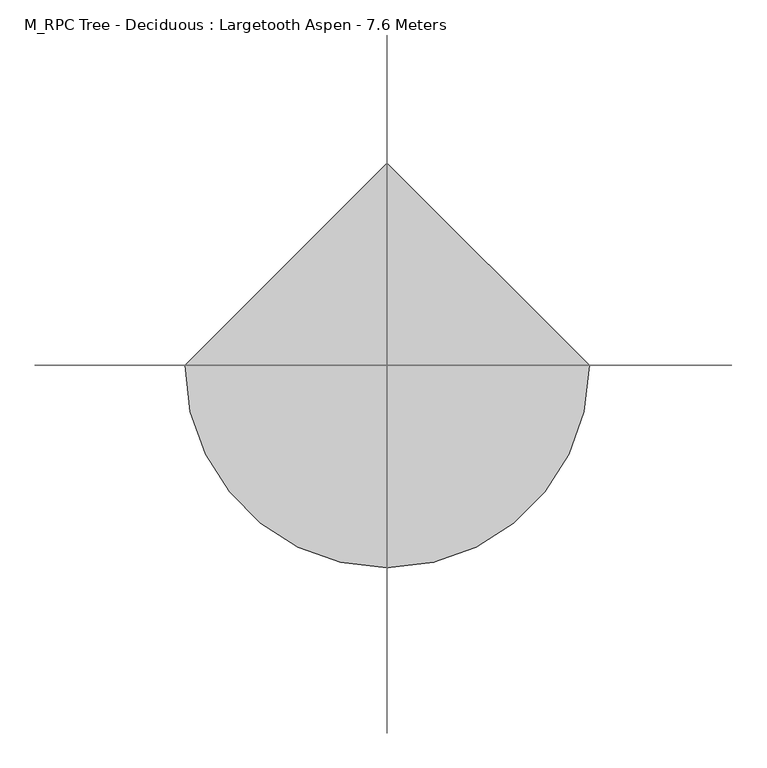
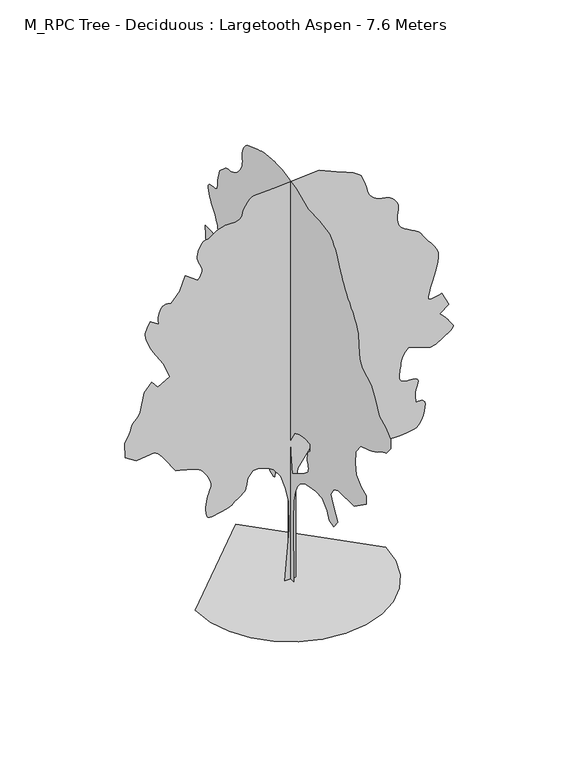
"""IFC4 building model written with IfcOpenShell, lengths in millimetres: geographic element geometry, M_RPC Tree - Deciduous : Largetooth Aspen - 7.6 Meters."""

from ifc_helpers import new_model, si_unit, origin, place, context, project, spatial, triangles, source, transform, mapped, element, save


def m_rpc_tree_deciduous_largetooth_aspen_7_6_meters_7a32e79d(model_context):
    return source(origin(), model_context, "Body", "Tessellation", [
        triangles([(92.8617737, 0.000406, 0.005513), (-103.915959, 0.000406, 0.005513), (-22.8901635, 0.0003494, 949.168154), (-34.4652064, 0.0003176, 1481.626133), (-92.3406663, 0.0003011, 1759.4311237), (-173.3674883, 0.0002866, 2002.5093098), (-300.6937099, 0.0002762, 2176.1362118), (-404.8693279, 0.0002728, 2234.0127663), (-566.9214277, 0.0002694, 2291.8891754), (-682.6743914, 0.0002694, 2291.8891754), (-763.7004776, 0.0002762, 2176.1362118), (-798.427355, 0.0002852, 2025.6589142), (-801.2950579, 0.0002863, 2008.1460297), (-806.4934324, 0.0002874, 1989.7185207), (-816.3455927, 0.0002886, 1969.4722275), (-833.1871519, 0.0002899, 1946.489764), (-859.3387533, 0.0002915, 1919.8644997), (-897.1360102, 0.0002934, 1888.6816647), (-948.9046526, 0.0002956, 1852.0320122), (-998.3097038, 0.0002977, 1817.003627), (-1032.3247061, 0.0002993, 1790.0718407), (-1058.2431822, 0.0003005, 1769.4200489), (-1083.3510246, 0.0003015, 1753.2220551), (-1114.9365967, 0.0003023, 1739.6560226), (-1160.2933485, 0.000303, 1726.8980804), (-1226.7072453, 0.0003038, 1713.1294441), (-1299.8367931, 0.0003048, 1697.5064152), (-1361.0192505, 0.0003056, 1683.0943588), (-1411.0653236, 0.0003062, 1673.9516029), (-1450.7854282, 0.0003062, 1674.1187439), (-1480.9902706, 0.0003054, 1687.6517841), (-1502.4856155, 0.0003035, 1718.5964069), (-1516.0869656, 0.0003004, 1771.0059986), (-1522.0251205, 0.0002967, 1833.4045155), (-1521.0802654, 0.0002932, 1891.7521168), (-1514.8710514, 0.00029, 1946.2541679), (-1505.0164204, 0.0002869, 1997.1108021), (-1493.1376396, 0.0002841, 2044.5246231), (-1480.8535057, 0.0002815, 2088.6983803), (-1469.7852859, 0.000279, 2129.8371483), (-1458.1775642, 0.0002769, 2165.8103886), (-1444.9485752, 0.000275, 2196.5194153), (-1432.7328964, 0.0002733, 2225.2042923), (-1424.1600185, 0.0002715, 2255.1052288), (-1421.8648098, 0.0002695, 2289.4596725), (-1428.479377, 0.000267, 2331.5079781), (-1446.6358269, 0.0002638, 2384.4900639), (-1473.3978561, 0.0002604, 2441.7913628), (-1503.3976238, 0.0002573, 2494.2338013), (-1535.6266159, 0.0002545, 2541.2094223), (-1569.0690514, 0.0002521, 2582.1229134), (-1602.7142361, 0.00025, 2616.3228607), (-1635.5487144, 0.0002484, 2643.2520309), (-1666.5644085, 0.0002473, 2662.3026123), (-1701.7269424, 0.0002464, 2677.1732162), (-1746.6125748, 0.0002455, 2692.0694), (-1799.5946606, 0.0002446, 2706.940004), (-1859.0570194, 0.0002437, 2721.8358971), (-1923.3782387, 0.0002428, 2736.706501), (-1990.9396671, 0.000242, 2751.5773956), (-2060.1198921, 0.0002411, 2766.4732887), (-2256.8962532, 0.0002238, 3055.8556252), (-2301.7818855, 0.0002202, 3116.5289566), (-2338.160479, 0.0002175, 3161.4195305), (-2367.4508423, 0.0002156, 3193.1367805), (-2391.0741096, 0.0002144, 3214.3154297), (-2410.4440029, 0.0002136, 3227.61549), (-2426.9816563, 0.0002131, 3235.6461044), (-2442.1006462, 0.0002128, 3241.041996), (-2766.1945267, 0.0002148, 3206.3353935), (-2962.9836777, 0.0002073, 3333.6607613), (-2974.5611687, 0.0001914, 3599.8884064), (-2952.3436295, 0.000189, 3639.5351143), (-2930.8612198, 0.0001867, 3678.9789276), (-2910.7717484, 0.0001843, 3718.0431129), (-2892.8103447, 0.0001821, 3756.473616), (-2877.7118477, 0.0001798, 3794.0937035), (-2866.1343567, 0.0001776, 3830.70019), (-2858.8132919, 0.0001755, 3866.1160515), (-2847.3878265, 0.0001735, 3899.5814507), (-2825.6772331, 0.0001716, 3931.2481224), (-2797.4559906, 0.0001698, 3962.0787987), (-2766.6000252, 0.0001679, 3993.137368), (-2736.9852631, 0.000166, 4025.3865623), (-2712.4120537, 0.000164, 4059.8905609), (-2696.7560326, 0.0001617, 4097.611805), (-2627.2919586, 0.000141, 4444.881015), (-2488.4021805, 0.0001321, 4595.3354942), (-2384.2240917, 0.0001396, 4468.0101265), (-2164.2955101, 0.0001327, 4583.7835831), (-2280.0484737, 0.0001155, 4873.1406303), (-2465.2501053, 9.82e-05, 5162.5226761), (-2487.5231644, 9.58e-05, 5203.6643509), (-2513.0364326, 9.27e-05, 5254.9385468), (-2539.3601166, 8.93e-05, 5312.268187), (-2564.0600624, 8.58e-05, 5371.6238663), (-2584.7067673, 8.24e-05, 5428.9535065), (-2598.8934013, 7.93e-05, 5480.2277023), (-2604.1628471, 7.69e-05, 5521.3693771), (-2601.4519661, 7.48e-05, 5555.7463486), (-2593.9027176, 7.28e-05, 5589.5413788), (-2582.2746483, 7.08e-05, 5622.8038834), (-2567.4293335, 6.89e-05, 5655.6611801), (-2550.1521904, 6.69e-05, 5688.2394241), (-2531.2585762, 6.5e-05, 5720.5903564), (-2511.5516396, 6.31e-05, 5752.8651306), (-2361.0744873, 6.93e-05, 5648.6941635), (-2365.8675087, 6.73e-05, 5681.019516), (-2369.6472198, 6.54e-05, 5713.8518143), (-2371.4003105, 6.34e-05, 5747.6968414), (-2370.118412, 6.13e-05, 5783.0621246), (-2364.7857433, 5.9e-05, 5820.4540283), (-2354.391465, 5.67e-05, 5860.3794983), (-2337.9248829, 5.41e-05, 5903.344899), (-2316.394075, 5.19e-05, 5940.9141174), (-2291.8258072, 5.04e-05, 5965.7155106), (-2264.7268799, 4.95e-05, 5979.8768555), (-2235.6036575, 4.92e-05, 5985.5515091), (-2204.9604698, 4.92e-05, 5984.8422501), (-2173.3064426, 4.95e-05, 5979.8768555), (-2141.1459057, 5e-05, 5972.7836838), (-1990.6686081, 3.96e-05, 6146.4178528), (-1886.4929901, 2.44e-05, 6401.0685883), (-1666.5644085, 3.41e-05, 6239.0110382), (-1644.4939533, 3.23e-05, 6268.8284042), (-1623.9409927, 3.05e-05, 6298.823085), (-1606.4256374, 2.87e-05, 6329.2229736), (-1593.4675621, 2.69e-05, 6360.2309647), (-1586.584552, 2.5e-05, 6392.0749512), (-1587.2913403, 2.3e-05, 6424.9066681), (-1597.1131245, 2.1e-05, 6458.9551712), (-1613.1085144, 1.89e-05, 6493.7885101), (-1630.1173599, 1.68e-05, 6529.2043716), (-1646.3154991, 1.46e-05, 6565.8614365), (-1659.8813862, 1.23e-05, 6604.3428085), (-1668.993766, 9.9e-06, 6645.2310104), (-1671.8286221, 7.3e-06, 6689.1585617), (-1666.5644085, 4.4e-06, 6736.759726), (-1653.9432312, 1.5e-06, 6785.3747818), (-1636.4607227, -1.2e-06, 6830.974324), (-1614.9300602, -3.6e-06, 6871.9131042), (-1590.1616592, -5.7e-06, 6906.5691284), (-1562.9612846, -7.3e-06, 6933.3209839), (-1534.1394974, -8.3e-06, 6950.5728378), (-1504.512236, -8.7e-06, 6956.6782791), (-1471.3382435, -9.2e-06, 6965.0132355), (-1431.8891979, -1.05e-05, 6986.521225), (-1386.9707188, -1.22e-05, 7015.9078033), (-1337.3959831, -1.41e-05, 7047.9291046), (-1283.9756973, -1.59e-05, 7077.315683), (-1227.5178062, -1.72e-05, 7098.8236725), (-1168.8306908, -1.77e-05, 7107.1580475), (-1109.0314339, -1.76e-05, 7106.8289978), (-1050.4481638, -1.77e-05, 7107.2847839), (-995.7104439, -1.79e-05, 7110.8060806), (-947.4530697, -1.84e-05, 7119.5718246), (-908.3055319, -1.94e-05, 7135.8353668), (-880.9024807, -2.09e-05, 7161.8273849), (-867.8760956, -2.32e-05, 7199.7512329), (-856.9422426, -2.61e-05, 7248.5941818), (-835.6824938, -2.93e-05, 7302.6809967), (-806.5264246, -3.26e-05, 7357.4009125), (-771.9008492, -3.56e-05, 7408.0420074), (-734.2403572, -3.81e-05, 7449.9940979), (-695.9718355, -3.98e-05, 7478.5696793), (-659.5247869, -4.04e-05, 7489.1341507), (-323.8458215, -4.18e-05, 7512.2885513), (509.5693688, -4.53e-05, 7570.1751343), (926.2744205, -3.42e-05, 7384.9631836), (995.3532709, -3.26e-05, 7357.5526474), (1062.2079111, -3.09e-05, 7329.4578506), (1124.6038118, -2.92e-05, 7299.9195374), (1180.3219225, -2.73e-05, 7268.2778641), (1227.1277138, -2.52e-05, 7233.7741562), (1262.7970482, -2.29e-05, 7195.7485703), (1285.1055702, -2.04e-05, 7153.4674301), (1299.9533558, -1.79e-05, 7111.9461273), (1314.5985374, -1.58e-05, 7075.1117477), (1328.8409821, -1.37e-05, 7040.4813034), (1342.4753242, -1.16e-05, 7005.6479645), (1355.2991055, -9.4e-06, 6968.1799026), (1367.1094311, -6.8e-06, 6925.6702881), (1377.7063133, -3.9e-06, 6875.662294), (1393.5345623, -8e-07, 6823.9573105), (1419.2834267, 2e-06, 6778.1292938), (1452.117905, 4.3e-06, 6738.3811386), (1489.2059029, 6.3e-06, 6704.890741), (1527.709948, 7.9e-06, 6677.9109924), (1564.7979458, 9.1e-06, 6657.5936279), (1597.6348949, 9.9e-06, 6644.1415421), (1628.0070236, 1.04e-05, 6636.0856384), (1659.1872425, 1.07e-05, 6630.6638763), (1690.5726814, 1.1e-05, 6626.2310074), (1721.5527672, 1.13e-05, 6621.2150345), (1751.5195427, 1.17e-05, 6613.9439667), (1779.8675217, 1.24e-05, 6602.8481323), (1805.9862762, 1.34e-05, 6586.2799576), (1831.2638031, 1.47e-05, 6563.7586578), (1856.5388592, 1.63e-05, 6536.6015945), (1880.3977226, 1.82e-05, 6505.7964981), (1901.4218754, 2.02e-05, 6472.3560974), (1918.1949795, 2.23e-05, 6437.2948654), (1929.2986622, 2.44e-05, 6401.625531), (1933.3139694, 2.65e-05, 6366.3364059), (1929.8053173, 2.9e-05, 6325.1191544), (1922.245895, 3.2e-05, 6273.1351181), (1915.0916805, 3.56e-05, 6213.8805954), (1912.7964718, 3.93e-05, 6150.775145), (1919.8163921, 4.31e-05, 6087.2644867), (1940.6048035, 4.67e-05, 6026.7937592), (1979.615649, 5e-05, 5972.7836838), (2034.2165314, 5.26e-05, 5927.5631882), (2096.1082478, 5.5e-05, 5888.8289246), (2161.2403187, 5.71e-05, 5853.1340103), (2225.5615379, 5.92e-05, 5817.0088898), (2285.0238968, 6.16e-05, 5777.0584213), (2335.5764797, 6.44e-05, 5729.8118866), (2373.1711327, 6.79e-05, 5671.8491455), (2411.6423309, 7.17e-05, 5607.2240204), (2462.6659607, 7.56e-05, 5541.7878983), (2518.9567108, 7.96e-05, 5474.7303635), (2573.2307236, 8.38e-05, 5405.2415817), (2618.1721664, 8.81e-05, 5332.5093933), (2646.5201454, 9.27e-05, 5255.7495438), (2650.9785942, 9.76e-05, 5174.1004578), (2634.6386032, 0.0001032, 5079.7841217), (2608.190799, 0.0001097, 4970.8762344), (2575.6628426, 0.0001165, 4855.508567), (2541.0826859, 0.0001233, 4741.7367325), (2508.5625778, 0.0001295, 4637.6927925), (2482.1043091, 0.0001347, 4551.4835197), (2465.7718758, 0.0001383, 4491.1648178), (2464.9611694, 0.0001404, 4454.9635391), (2480.5538223, 0.0001417, 4433.9369156), (2509.8113388, 0.0001422, 4425.5769608), (2550.0001648, 0.0001421, 4427.3248192), (2598.3867462, 0.0001415, 4436.6727951), (2652.2453773, 0.0001407, 4451.0876129), (2708.839888, 0.0001396, 4468.0101265), (2836.1652557, 0.0001548, 4213.3596817), (2674.1332855, 0.0001624, 4086.0346046), (2698.8841003, 0.0001637, 4063.6400414), (2723.4573097, 0.0001651, 4040.7132431), (2747.6253113, 0.0001665, 4016.7987144), (2771.1852104, 0.0001681, 3991.3386406), (2793.9346939, 0.0001697, 3963.8775261), (2815.6705765, 0.0001715, 3933.8828453), (2836.1652557, 0.0001735, 3900.8482338), (2858.1037422, 0.0001754, 3868.6749069), (2881.2584335, 0.000177, 3840.554821), (2901.1705902, 0.0001786, 3814.8921432), (2913.3811821, 0.0001801, 3790.0148827), (2913.4570496, 0.0001816, 3764.3269157), (2896.9144547, 0.0001833, 3736.2324097), (2859.3199471, 0.0001852, 3704.0590828), (2604.6695023, 0.0001955, 3530.4246231), (2500.4962097, 0.0001962, 3518.8471321), (2118.5182171, 0.0001886, 3646.1724998), (2091.3836815, 0.0001903, 3618.7110947), (2065.163625, 0.000192, 3590.1352226), (2040.7651142, 0.0001938, 3559.3298355), (2019.0975414, 0.0001958, 3525.1551773), (2001.0780018, 0.0001981, 3486.5726486), (1987.6134167, 0.0002008, 3442.3913338), (1979.615649, 0.0002038, 3391.5220551), (1974.0473843, 0.0002068, 3342.1474525), (1967.6684132, 0.0002092, 3301.2848305), (1961.0868382, 0.0002113, 3266.096862), (1954.9106163, 0.0002132, 3233.7209312), (1949.7477047, 0.0002151, 3201.3702896), (1946.2035896, 0.0002172, 3166.1567413), (1944.888699, 0.0002197, 3125.2941193), (1953.8643139, 0.000222, 3086.7368797), (1977.0163891, 0.0002236, 3059.0981598), (2008.6704163, 0.0002247, 3040.5542336), (2043.1591541, 0.0002254, 3029.3316628), (2074.8131813, 0.0002257, 3023.5555618), (2097.9652565, 0.0002259, 3021.4277847), (2106.9408714, 0.0002259, 3021.1237335), (2119.5973663, 0.0002258, 3022.0103073), (2151.4869896, 0.0002258, 3022.4663841), (2193.5021576, 0.000226, 3019.2997169), (2236.5307812, 0.0002266, 3009.242482), (2271.4578644, 0.0002278, 2989.0771431), (2289.1759689, 0.0002298, 2955.5102966), (2280.5702442, 0.0002328, 2905.3758568), (2259.8146797, 0.0002362, 2847.8691925), (2246.3500946, 0.0002394, 2794.0105614), (2238.9578133, 0.0002425, 2743.191861), (2236.4270084, 0.0002453, 2694.7799904), (2237.5416206, 0.0002481, 2648.2174255), (2241.0857357, 0.0002508, 2602.8707748), (2245.8434395, 0.0002535, 2558.1069374), (2285.1910378, 0.0002532, 2562.540097), (2322.5171024, 0.0002531, 2563.730722), (2355.7899261, 0.0002535, 2558.4106979), (2382.9903008, 0.0002544, 2543.4133575), (2402.0916058, 0.000256, 2515.4278564), (2411.0672207, 0.0002587, 2471.2540993), (2407.8954666, 0.0002625, 2407.6396683), (2395.1731327, 0.0002668, 2334.9507912), (2376.983836, 0.0002708, 2266.9155544), (2353.5301804, 0.0002745, 2205.3632069), (2325.0124443, 0.0002777, 2152.110062), (2291.638464, 0.0002803, 2108.9801365), (2253.6054657, 0.0002821, 2077.7999176), (2211.1189602, 0.0002832, 2060.3858643), (2171.2620907, 0.0002837, 2051.7801395), (2137.4826118, 0.000284, 2045.4011684), (2104.5113686, 0.0002843, 2040.64361), (2067.0864727, 0.0002845, 2036.8967457), (2019.9412399, 0.0002847, 2033.5578506), (1957.8137821, 0.000285, 2030.0137356), (1875.4374149, 0.0002852, 2025.6589142), (1785.9069786, 0.0002851, 2027.1105698), (1704.880965, 0.0002844, 2040.1039627), (1630.9407108, 0.000283, 2062.7139198), (1562.6724941, 0.0002812, 2093.0175934), (1498.6551807, 0.0002791, 2129.0947517), (1437.4727234, 0.0002767, 2169.0176056), (1377.7063133, 0.0002742, 2210.8631618), (1123.0508543, 0.0002597, 2453.9412025), (856.8231365, 0.0002528, 2569.6841377), (544.2937391, 0.0002542, 2546.5547356), (393.8164052, 0.0002611, 2430.7917435), (289.6407872, 0.00027, 2280.3144459), (127.5871523, 0.0002838, 2048.8109894), (92.8617737, 0.0003011, 1759.4311237), (92.8617737, 0.0003383, 1134.3723289), (-0.0023646, 90.6053344, 1.1e-05), (-0.0023646, -94.5971056, 0.0), (-0.0023646, -83.0220672, 1157.5168465), (-0.0023646, -94.5971056, 1527.9227257), (-0.0023646, -140.8980313, 1724.6992321), (-0.0023646, -210.3490428, 1875.1765297), (-0.0023646, -302.9508941, 1990.9294933), (-0.0023646, -441.853444, 2071.9555069), (-0.0023646, -557.6038642, 2095.1051113), (-0.0023646, -789.1072117, 2141.4067909), (-0.0023646, -985.8861889, 2129.8320614), (-0.0023646, -1136.3635592, 1979.3547638), (-0.0023646, -1205.8147705, 1840.4521957), (-0.0023646, -1333.1399929, 1794.1505161), (-0.0023646, -1472.042561, 1967.7774181), (-0.0023646, -1321.5652634, 2199.2833454), (-0.0023646, -1252.1139793, 2361.3353725), (-0.0023646, -1333.1399929, 2500.2354698), (-0.0023646, -1483.6172905, 2569.6841377), (-0.0023646, -1969.7736626, 2569.6841377), (-0.0023646, -2351.7542713, 2835.9117828), (-0.0023646, -2351.7542713, 2997.9690422), (-0.0023646, -2189.7022442, 3067.4075363), (-0.0023646, -2039.2249466, 3206.3101044), (-0.0023646, -2004.5006126, 3403.0992554), (-0.0023646, -2027.6500717, 3634.5950089), (-0.0023646, -2178.1273693, 3831.3841599), (-0.0023646, -2444.3551598, 3923.9773453), (-0.0023646, -2488.9367409, 3941.4068047), (-0.0023646, -2533.110498, 3959.1147354), (-0.0023646, -2576.4735489, 3977.4307686), (-0.0023646, -2618.6279526, 3996.6839539), (-0.0023646, -2659.1612343, 4017.1280548), (-0.0023646, -2697.6678955, 4039.0921211), (-0.0023646, -2733.7427284, 4062.8799133), (-0.0023646, -2768.4493309, 4086.3386559), (-0.0023646, -2803.1812225, 4107.3652794), (-0.0023646, -2837.9131142, 4126.3652824), (-0.0023646, -2872.6450058, 4143.7438728), (-0.0023646, -2907.351899, 4159.9065491), (-0.0023646, -2942.0837906, 4175.258519), (-0.0023646, -2976.8156822, 4190.2052811), (-0.0023646, -3104.14105, 4352.2622498), (-0.0023646, -3104.14105, 4514.3195091), (-0.0023646, -2953.6609909, 4653.2220772), (-0.0023646, -2756.8971291, 4757.3927536), (-0.0023646, -2629.5467628, 5000.4657074), (-0.0023646, -2502.234185, 5185.6776581), (-0.0023646, -2224.4291943, 5336.1574265), (-0.0023646, -2143.4030354, 5463.4827942), (-0.0023646, -2120.2509602, 5718.1329483), (-0.0023646, -2097.1013557, 5926.4743011), (-0.0023646, -2072.264645, 5978.4327576), (-0.0023646, -2047.225185, 6029.4540619), (-0.0023646, -2021.7779011, 6078.651059), (-0.0023646, -1995.7251308, 6125.1127579), (-0.0023646, -1968.8641251, 6167.9514221), (-0.0023646, -1940.9873383, 6206.2043198), (-0.0023646, -1911.8997242, 6239.0110382), (-0.0023646, -1875.8225658, 6277.7964615), (-0.0023646, -1830.2327614, 6330.9455429), (-0.0023646, -1779.7788643, 6393.0121033), (-0.0023646, -1729.1274502, 6458.4988037), (-0.0023646, -1682.9270725, 6521.9844635), (-0.0023646, -1645.83922, 6577.9705811), (-0.0023646, -1622.5198586, 6620.9865601), (-0.0023646, -1605.6807701, 6657.1372604), (-0.0023646, -1585.6016178, 6696.1255783), (-0.0023646, -1563.2930958, 6737.9253525), (-0.0023646, -1539.7736012, 6782.5877426), (-0.0023646, -1516.0490318, 6830.0627518), (-0.0023646, -1493.1350235, 6880.3742157), (-0.0023646, -1472.042561, 6933.5238785), (-0.0023646, -1448.8245014, 6986.749118), (-0.0023646, -1419.5316673, 7037.5425293), (-0.0023646, -1385.1772236, 7086.3087387), (-0.0023646, -1346.7743351, 7133.4541168), (-0.0023646, -1305.3316612, 7179.3832901), (-0.0023646, -1261.8673084, 7224.5020477), (-0.0023646, -1217.3895727, 7269.2155975), (-0.0023646, -893.2828297, 7327.0766006), (-0.0023646, -546.029062, 7338.653801), (-0.0023646, -175.623419, 7500.711351), (-0.0023646, 264.2314734, 7593.3045364), (-0.0023646, 323.6937959, 7595.7363647), (-0.0023646, 382.7508379, 7597.8647232), (-0.0023646, 440.9996807, 7599.3843979), (-0.0023646, 498.0300296, 7599.9925003), (-0.0023646, 553.4441254, 7599.3843979), (-0.0023646, 606.831528, 7597.2566208), (-0.0023646, 657.7895004, 7593.3045364), (-0.0023646, 706.7891985, 7588.2379852), (-0.0023646, 754.9781902, 7582.5883301), (-0.0023646, 802.9670488, 7575.698053), (-0.0023646, 851.3612606, 7566.9828873), (-0.0023646, 900.7663118, 7555.8620544), (-0.0023646, 951.7900869, 7541.6751297), (-0.0023646, 1005.0433044, 7523.8657516), (-0.0023646, 1340.7248497, 7408.1181656), (-0.0023646, 1370.3545818, 7383.1138779), (-0.0023646, 1399.173753, 7356.8689682), (-0.0023646, 1426.3741276, 7328.2166473), (-0.0023646, 1451.1425285, 7295.9418732), (-0.0023646, 1472.6733364, 7258.7778625), (-0.0023646, 1490.1558449, 7215.5595703), (-0.0023646, 1502.7768768, 7165.019632), (-0.0023646, 1507.1292274, 7116.7342072), (-0.0023646, 1503.5851124, 7077.7714691), (-0.0023646, 1497.0060081, 7043.2421814), (-0.0023646, 1492.2458336, 7008.3076859), (-0.0023646, 1494.1711521, 6968.1293243), (-0.0023646, 1507.6358826, 6917.7916992), (-0.0023646, 1537.5012108, 6852.5078934), (-0.0023646, 1578.4019119, 6786.1851974), (-0.0023646, 1620.9238804, 6734.4546341), (-0.0023646, 1663.8485859, 6694.8587952), (-0.0023646, 1705.9652012, 6664.9908508), (-0.0023646, 1746.0576668, 6642.4189728), (-0.0023646, 1782.9075977, 6624.7107513), (-0.0023646, 1815.3063469, 6609.4093597), (-0.0023646, 1845.0703732, 6598.3135254), (-0.0023646, 1874.8345448, 6592.8923447), (-0.0023646, 1904.598571, 6590.2826202), (-0.0023646, 1934.3652134, 6587.699057), (-0.0023646, 1964.129385, 6582.2522964), (-0.0023646, 1993.8935566, 6571.1558807), (-0.0023646, 2023.6575829, 6551.5483566), (-0.0023646, 2197.2869556, 6401.0685883), (-0.0023646, 2266.7357689, 6181.1500351), (-0.0023646, 2264.4760231, 6146.5445892), (-0.0023646, 2263.5310226, 6112.7751389), (-0.0023646, 2265.2182743, 6080.6021027), (-0.0023646, 2270.8549942, 6050.8858932), (-0.0023646, 2281.7533115, 6024.3875107), (-0.0023646, 2299.23582, 6001.9417877), (-0.0023646, 2324.612178, 5984.3608841), (-0.0023646, 2359.9116222, 5974.3033585), (-0.0023646, 2402.9047829, 5970.5285889), (-0.0023646, 2448.5301956, 5967.9700241), (-0.0023646, 2491.7284309, 5961.5605316), (-0.0023646, 2527.4306122, 5946.2341415), (-0.0023646, 2550.5826874, 5916.9237213), (-0.0023646, 2556.1056061, 5868.6127167), (-0.0023646, 2547.4416, 5812.448703), (-0.0023646, 2532.0896301, 5762.3651321), (-0.0023646, 2511.1641632, 5717.3475311), (-0.0023646, 2485.7878052, 5676.3837524), (-0.0023646, 2457.0700813, 5638.4599045), (-0.0023646, 2426.1228424, 5602.562677), (-0.0023646, 2394.0634621, 5567.6531799), (-0.0023646, 2369.3610455, 5525.4987762), (-0.0023646, 2345.2664406, 5483.4705276), (-0.0023646, 2322.3854244, 5441.6201752), (-0.0023646, 2301.3284248, 5400.0732925), (-0.0023646, 2282.698312, 5358.9321991), (-0.0023646, 2267.1081299, 5318.2974701), (-0.0023646, 2255.160894, 5278.2708435), (-0.0023646, 2248.9518253, 5240.6254669), (-0.0023646, 2249.4254883, 5206.6025436), (-0.0023646, 2255.4649452, 5175.6201324), (-0.0023646, 2265.9605255, 5147.0695496), (-0.0023646, 2279.797617, 5120.3426926), (-0.0023646, 2295.861462, 5094.8320404), (-0.0023646, 2313.0374485, 5069.9294907), (-0.0023646, 2463.5147461, 5093.0844727), (-0.0023646, 2648.7240807, 5093.0844727), (-0.0023646, 2625.5693893, 4757.3927536), (-0.0023646, 2417.2130665, 4398.5716324), (-0.0023646, 2409.7574169, 4356.4422272), (-0.0023646, 2402.1979946, 4314.642453), (-0.0023646, 2394.4358231, 4273.4252014), (-0.0023646, 2386.3697456, 4233.1451019), (-0.0023646, 2377.898315, 4194.0559181), (-0.0023646, 2368.9227001, 4156.486409), (-0.0023646, 2359.3391281, 4120.7664963), (-0.0023646, 2344.9953815, 4082.1586784), (-0.0023646, 2323.9712288, 4037.2681046), (-0.0023646, 2299.5044083, 3988.3492882), (-0.0023646, 2274.8373093, 3937.5814568), (-0.0023646, 2253.2051994, 3887.2441223), (-0.0023646, 2237.8507587, 3839.5162216), (-0.0023646, 2232.0114349, 3796.6522682), (-0.0023646, 2236.7360012, 3758.6522621), (-0.0023646, 2249.9651356, 3723.6921867), (-0.0023646, 2270.279884, 3691.2656776), (-0.0023646, 2296.2641991, 3660.865789), (-0.0023646, 2326.5020336, 3631.9602859), (-0.0023646, 2359.5747242, 3604.0936729), (-0.0023646, 2394.0634621, 3576.7337151), (-0.0023646, 2706.5853745, 3646.1724998), (-0.0023646, 2723.8372284, 3596.6458717), (-0.0023646, 2740.3798233, 3547.4991623), (-0.0023646, 2755.5039001, 3499.1884483), (-0.0023646, 2768.4746201, 3452.0686501), (-0.0023646, 2778.6333023, 3406.5699738), (-0.0023646, 2785.245108, 3363.0979179), (-0.0023646, 2787.6266487, 3322.0832703), (-0.0023646, 2774.199852, 3282.9940865), (-0.0023646, 2739.6958534, 3244.7153183), (-0.0023646, 2692.8545265, 3206.6647339), (-0.0023646, 2642.3654572, 3168.1836525), (-0.0023646, 2596.9426483, 3128.7142593), (-0.0023646, 2565.3015564, 3087.5981644), (-0.0023646, 2556.1056061, 3044.2784248), (-0.0023646, 2564.4399811, 3002.6556747), (-0.0023646, 2578.8547989, 2966.5049744), (-0.0023646, 2598.3361679, 2934.9397499), (-0.0023646, 2621.8454887, 2906.9969788), (-0.0023646, 2648.4200294, 2881.7903778), (-0.0023646, 2676.9959015, 2858.3825043), (-0.0023646, 2706.5853745, 2835.9117828), (-0.0023646, 2776.0491577, 2604.4160294), (-0.0023646, 2709.3974121, 2602.1106468), (-0.0023646, 2644.6708397, 2600.945311), (-0.0023646, 2583.7949043, 2601.984201), (-0.0023646, 2528.6796638, 2606.3667824), (-0.0023646, 2481.2656975, 2615.2081032), (-0.0023646, 2443.468586, 2629.6226303), (-0.0023646, 2417.2130665, 2650.725412), (-0.0023646, 2391.9710026, 2676.8694557), (-0.0023646, 2357.0109272, 2705.4453278), (-0.0023646, 2313.9494568, 2736.0478203), (-0.0023646, 2264.407568, 2768.2973053), (-0.0023646, 2210.0068188, 2801.7371246), (-0.0023646, 2152.3684765, 2835.987941), (-0.0023646, 2093.1088669, 2870.6436745), (-0.0023646, 2090.6465172, 2833.3785072), (-0.0023646, 2088.2828533, 2795.8345779), (-0.0023646, 2086.1244095, 2757.6572571), (-0.0023646, 2084.2675461, 2718.5680733), (-0.0023646, 2082.8158905, 2678.2879738), (-0.0023646, 2081.8710354, 2636.4626198), (-0.0023646, 2081.5341373, 2592.838829), (-0.0023646, 2079.9481876, 2547.390731), (-0.0023646, 2074.514217, 2502.7332825), (-0.0023646, 2064.2212406, 2462.5418404), (-0.0023646, 2048.0560936, 2430.4471424), (-0.0023646, 2025.0077911, 2410.0995472), (-0.0023646, 1994.0631683, 2405.1366234), (-0.0023646, 1954.2062988, 2419.2093109), (-0.0023646, 1909.2219807, 2445.3635284), (-0.0023646, 1863.6321762, 2473.9469582), (-0.0023646, 1817.5331005, 2504.5546829), (-0.0023646, 1771.028817, 2536.7762627), (-0.0023646, 1724.222953, 2570.216082), (-0.0023646, 1677.2144852, 2604.4921875), (-0.0023646, 1630.1020992, 2639.147921), (-0.0023646, 1352.2995792, 2720.1639061), (-0.0023646, 1074.4945158, 2627.5707207), (-0.0023646, 900.8676138, 2419.2093109), (-0.0023646, 923.2420475, 2389.5794334), (-0.0023646, 945.9203871, 2360.7602623), (-0.0023646, 969.204213, 2333.5598877), (-0.0023646, 993.4000471, 2308.7916321), (-0.0023646, 1018.8119408, 2287.2608242), (-0.0023646, 1045.7412563, 2269.7783157), (-0.0023646, 1074.4945158, 2257.1572838), (-0.0023646, 1101.897567, 2244.8731499), (-0.0023646, 1125.0471714, 2228.3381126), (-0.0023646, 1144.6551315, 2208.258815), (-0.0023646, 1161.4257648, 2185.344952), (-0.0023646, 1176.07349, 2160.305492), (-0.0023646, 1189.3025517, 2133.8473686), (-0.0023646, 1201.8222816, 2106.6798409), (-0.0023646, 1169.4919149, 2099.1888737), (-0.0023646, 1136.6574366, 2091.3938553), (-0.0023646, 1102.8070318, 2082.9907345), (-0.0023646, 1067.4417486, 2073.6756054), (-0.0023646, 1030.0497723, 2063.1471783), (-0.0023646, 990.1269911, 2051.0986404), (-0.0023646, 947.1668226, 2037.2287022), (-0.0023646, 904.2091249, 2020.3237747), (-0.0023646, 864.2863438, 1999.7708141), (-0.0023646, 826.8943674, 1976.1830097), (-0.0023646, 791.5265408, 1950.1630863), (-0.0023646, 757.6786795, 1922.3217625), (-0.0023646, 724.8442011, 1893.2645245), (-0.0023646, 692.5138344, 1863.6018002), (-0.0023646, 692.5138344, 1701.5496277), (-0.0023646, 650.5998957, 1674.7216141), (-0.0023646, 610.2059223, 1650.6246838), (-0.0023646, 572.8469018, 1631.9970417), (-0.0023646, 540.0453429, 1621.5699165), (-0.0023646, 513.3187039, 1622.0765717), (-0.0023646, 494.1844431, 1636.2505611), (-0.0023646, 484.160055, 1666.8252937), (-0.0023646, 479.2682024, 1701.4811726), (-0.0023646, 474.7791232, 1728.6487003), (-0.0023646, 471.1007504, 1752.1706657), (-0.0023646, 468.638328, 1775.8927643), (-0.0023646, 467.7947385, 1803.6682491), (-0.0023646, 468.9752624, 1839.3374382), (-0.0023646, 472.5852528, 1886.7512592), (-0.0023646, 475.5214108, 1938.6212036), (-0.0023646, 474.812079, 1985.6298168), (-0.0023646, 471.0677945, 2028.5899853), (-0.0023646, 464.8915363, 2068.3100899), (-0.0023646, 456.893805, 2105.6006916), (-0.0023646, 447.6800869, 2141.2724968), (-0.0023646, 437.8608825, 2176.1311249), (-0.0023646, 241.0823958, 2187.7059998), (-0.0023646, 136.90626, 1990.9294933), (-0.0023646, 79.030296, 1655.2479481), (-0.0023646, 79.030296, 1226.9681305), (-0.0023646, 79.030296, 590.3344972), (-0.0022449, -48.2969385, 2025.6538273), (-0.0022449, -1.9959556, 2396.0597065), (-0.0022449, 9.5791323, 2615.9935204), (-0.0022449, -129.3229929, 2835.9117828), (-0.0022449, -279.801326, 2905.3758568), (-0.0022449, -453.4282099, 2928.5049683), (-0.0022449, -615.4803097, 2928.5049683), (-0.0022449, -615.4803097, 2789.62798), (-0.0022449, -534.4542598, 2720.1639061), (-0.0022449, -511.3046917, 2558.1069374), (-0.0022449, -521.1568156, 2548.0241226), (-0.0022449, -530.6061298, 2536.9282883), (-0.0022449, -539.2448104, 2523.7927528), (-0.0022449, -546.6699749, 2507.6277512), (-0.0022449, -552.4738358, 2487.4115433), (-0.0022449, -556.2535832, 2462.1366325), (-0.0022449, -557.6038642, 2430.7841858), (-0.0022449, -554.2294335, 2398.4207542), (-0.0022449, -544.7801193, 2370.3109875), (-0.0022449, -530.2691955, 2345.7427197), (-0.0022449, -511.7075014, 2324.0093079), (-0.0022449, -490.1108545, 2304.4038185), (-0.0022449, -466.4875508, 2286.2145218), (-0.0022449, -441.853444, 2268.7320133), (-1707.3661331, 0.0, 0.0031185), (-1662.2297894, -391.2146745, 0.0030952), (-1533.678479, -750.4840605, 0.0030738), (-1332.01012, -1067.5126745, 0.0030549), (-1067.5126745, -1332.01012, 0.0030391), (-750.4840605, -1533.678479, 0.0030271), (-391.2146745, -1662.2297894, 0.0030194), (7.48e-05, -1707.3661331, 0.0030167), (391.2146745, -1662.2297894, 0.0030194), (750.4840605, -1533.678479, 0.0030271), (1067.5126745, -1332.01012, 0.0030391), (1332.01012, -1067.5126745, 0.0030549), (1533.678479, -750.4840605, 0.0030738), (1662.2297894, -391.2146745, 0.0030952), (1707.3661331, 0.0001493, 0.0031185), (-0.0002245, 1707.3661331, 0.0032203)], [[122, 123, 124], [87, 88, 89], [1, 2, 3], [329, 1, 3], [329, 3, 4], [328, 329, 4], [328, 4, 5], [105, 106, 107], [327, 328, 5], [327, 5, 6], [104, 105, 107], [238, 239, 240], [238, 240, 241], [237, 238, 241], [236, 237, 241], [103, 104, 107], [86, 87, 89], [235, 236, 241], [102, 103, 107], [101, 102, 107], [100, 101, 107], [99, 100, 107], [98, 99, 107], [97, 98, 107], [96, 97, 107], [327, 6, 7], [326, 327, 7], [95, 96, 107], [70, 71, 72], [69, 70, 72], [69, 72, 73], [69, 73, 74], [69, 74, 75], [69, 75, 76], [69, 76, 77], [69, 77, 78], [94, 95, 107], [234, 235, 241], [93, 94, 107], [69, 78, 79], [69, 79, 80], [69, 80, 81], [69, 81, 82], [69, 82, 83], [69, 83, 84], [69, 84, 85], [68, 69, 85], [325, 326, 7], [325, 7, 8], [67, 68, 85], [92, 93, 107], [91, 92, 107], [60, 61, 62], [67, 85, 86], [67, 86, 89], [67, 89, 90], [66, 67, 90], [65, 66, 90], [64, 65, 90], [63, 64, 90], [62, 63, 90], [60, 62, 90], [59, 60, 90], [58, 59, 90], [57, 58, 90], [56, 57, 90], [55, 56, 90], [54, 55, 90], [53, 54, 90], [284, 285, 286], [283, 284, 286], [282, 283, 286], [282, 286, 287], [281, 282, 287], [280, 281, 287], [279, 280, 287], [279, 287, 288], [278, 279, 288], [277, 278, 288], [277, 288, 289], [276, 277, 289], [275, 276, 289], [275, 289, 290], [52, 53, 90], [325, 8, 9], [121, 122, 124], [275, 290, 291], [30, 31, 32], [29, 30, 32], [29, 32, 33], [28, 29, 33], [28, 33, 34], [27, 28, 34], [27, 34, 35], [27, 35, 36], [26, 27, 36], [26, 36, 37], [26, 37, 38], [25, 26, 38], [25, 38, 39], [24, 25, 39], [23, 24, 39], [22, 23, 39], [21, 22, 39], [20, 21, 39], [20, 39, 40], [20, 40, 41], [20, 41, 42], [19, 20, 42], [19, 42, 43], [18, 19, 43], [18, 43, 44], [17, 18, 44], [16, 17, 44], [15, 16, 44], [14, 15, 44], [13, 14, 44], [12, 13, 44], [11, 12, 44], [11, 44, 45], [11, 45, 46], [10, 11, 46], [10, 46, 47], [10, 47, 48], [10, 48, 49], [10, 49, 50], [10, 50, 51], [252, 253, 254], [251, 252, 254], [251, 254, 255], [250, 251, 255], [249, 250, 255], [249, 255, 256], [248, 249, 256], [247, 248, 256], [246, 247, 256], [245, 246, 256], [245, 256, 257], [245, 257, 258], [244, 245, 258], [243, 244, 258], [242, 243, 258], [241, 242, 258], [234, 241, 258], [233, 234, 258], [274, 275, 291], [324, 325, 9], [51, 52, 90], [10, 51, 90], [9, 10, 90], [324, 9, 90], [323, 324, 90], [323, 90, 91], [323, 91, 107], [323, 107, 108], [323, 108, 109], [323, 109, 110], [323, 110, 111], [323, 111, 112], [323, 112, 113], [323, 113, 114], [323, 114, 115], [323, 115, 116], [323, 116, 117], [323, 117, 118], [323, 118, 119], [323, 119, 120], [323, 120, 121], [323, 121, 124], [323, 124, 125], [323, 125, 126], [323, 126, 127], [323, 127, 128], [323, 128, 129], [322, 323, 129], [322, 129, 130], [167, 168, 169], [274, 291, 292], [296, 297, 298], [296, 298, 299], [295, 296, 299], [294, 295, 299], [294, 299, 300], [293, 294, 300], [293, 300, 301], [293, 301, 302], [293, 302, 303], [293, 303, 304], [293, 304, 305], [293, 305, 306], [293, 306, 307], [293, 307, 308], [293, 308, 309], [293, 309, 310], [293, 310, 311], [293, 311, 312], [293, 312, 313], [293, 313, 314], [293, 314, 315], [293, 315, 316], [293, 316, 317], [293, 317, 318], [293, 318, 319], [292, 293, 319], [274, 292, 319], [274, 319, 320], [274, 320, 321], [274, 321, 322], [273, 274, 322], [273, 322, 130], [272, 273, 130], [271, 272, 130], [270, 271, 130], [269, 270, 130], [268, 269, 130], [267, 268, 130], [266, 267, 130], [265, 266, 130], [264, 265, 130], [263, 264, 130], [262, 263, 130], [261, 262, 130], [260, 261, 130], [259, 260, 130], [258, 259, 130], [233, 258, 130], [232, 233, 130], [231, 232, 130], [230, 231, 130], [229, 230, 130], [228, 229, 130], [227, 228, 130], [226, 227, 130], [225, 226, 130], [224, 225, 130], [223, 224, 130], [222, 223, 130], [221, 222, 130], [220, 221, 130], [219, 220, 130], [218, 219, 130], [217, 218, 130], [216, 217, 130], [215, 216, 130], [214, 215, 130], [213, 214, 130], [212, 213, 130], [211, 212, 130], [210, 211, 130], [209, 210, 130], [208, 209, 130], [207, 208, 130], [206, 207, 130], [205, 206, 130], [204, 205, 130], [203, 204, 130], [202, 203, 130], [201, 202, 130], [200, 201, 130], [199, 200, 130], [198, 199, 130], [197, 198, 130], [196, 197, 130], [195, 196, 130], [194, 195, 130], [193, 194, 130], [192, 193, 130], [191, 192, 130], [190, 191, 130], [189, 190, 130], [188, 189, 130], [187, 188, 130], [186, 187, 130], [185, 186, 130], [184, 185, 130], [183, 184, 130], [182, 183, 130], [181, 182, 130], [180, 181, 130], [179, 180, 130], [178, 179, 130], [177, 178, 130], [176, 177, 130], [175, 176, 130], [174, 175, 130], [173, 174, 130], [172, 173, 130], [171, 172, 130], [170, 171, 130], [169, 170, 130], [167, 169, 130], [167, 130, 131], [167, 131, 132], [167, 132, 133], [167, 133, 134], [167, 134, 135], [167, 135, 136], [164, 165, 166], [164, 166, 167], [163, 164, 167], [162, 163, 167], [161, 162, 167], [160, 161, 167], [159, 160, 167], [158, 159, 167], [143, 144, 145], [142, 143, 145], [141, 142, 145], [140, 141, 145], [140, 145, 146], [139, 140, 146], [138, 139, 146], [137, 138, 146], [136, 137, 146], [136, 146, 147], [136, 147, 148], [136, 148, 149], [136, 149, 150], [136, 150, 151], [136, 151, 152], [136, 152, 153], [136, 153, 154], [136, 154, 155], [136, 155, 156], [157, 158, 167], [157, 167, 136], [157, 136, 156], [634, 330, 635], [633, 634, 635], [632, 633, 635], [631, 632, 635], [540, 541, 542], [592, 593, 594], [494, 495, 496], [635, 330, 331], [635, 331, 332], [635, 332, 333], [635, 333, 334], [635, 334, 335], [658, 635, 335], [658, 335, 336], [658, 336, 337], [658, 337, 338], [540, 542, 543], [657, 658, 338], [631, 635, 636], [630, 631, 636], [518, 519, 520], [656, 657, 338], [656, 338, 339], [655, 656, 339], [654, 655, 339], [653, 654, 339], [540, 543, 544], [539, 540, 544], [518, 520, 521], [539, 544, 545], [538, 539, 545], [538, 545, 546], [538, 546, 547], [538, 547, 548], [537, 538, 548], [537, 548, 549], [536, 537, 549], [536, 549, 550], [536, 550, 551], [535, 536, 551], [535, 551, 552], [534, 535, 552], [493, 494, 496], [493, 496, 497], [343, 344, 345], [342, 343, 345], [341, 342, 345], [340, 341, 345], [340, 345, 346], [534, 552, 553], [533, 534, 553], [518, 521, 522], [350, 351, 352], [349, 350, 352], [349, 352, 353], [348, 349, 353], [533, 553, 554], [652, 653, 339], [518, 522, 523], [518, 523, 524], [533, 554, 555], [532, 533, 555], [518, 524, 525], [518, 525, 526], [518, 526, 527], [518, 527, 528], [518, 528, 529], [518, 529, 530], [518, 530, 531], [518, 531, 532], [518, 532, 555], [517, 518, 555], [516, 517, 555], [515, 516, 555], [607, 608, 609], [591, 592, 594], [591, 594, 595], [590, 591, 595], [590, 595, 596], [589, 590, 596], [588, 589, 596], [588, 596, 597], [587, 588, 597], [586, 587, 597], [586, 597, 598], [585, 586, 598], [585, 598, 599], [584, 585, 599], [584, 599, 600], [583, 584, 600], [583, 600, 601], [582, 583, 601], [514, 515, 555], [643, 644, 645], [630, 636, 637], [629, 630, 637], [581, 582, 601], [581, 601, 602], [348, 353, 354], [580, 581, 602], [580, 602, 603], [579, 580, 603], [651, 652, 339], [651, 339, 340], [651, 340, 346], [650, 651, 346], [649, 650, 346], [649, 346, 347], [648, 649, 347], [647, 648, 347], [646, 647, 347], [372, 373, 374], [371, 372, 374], [370, 371, 374], [369, 370, 374], [369, 374, 375], [368, 369, 375], [367, 368, 375], [366, 367, 375], [365, 366, 375], [364, 365, 375], [363, 364, 375], [362, 363, 375], [361, 362, 375], [360, 361, 375], [359, 360, 375], [358, 359, 375], [357, 358, 375], [356, 357, 375], [356, 375, 376], [356, 376, 377], [356, 377, 378], [645, 646, 347], [643, 645, 347], [642, 643, 347], [641, 642, 347], [641, 347, 348], [641, 348, 354], [641, 354, 355], [607, 609, 610], [513, 514, 555], [579, 603, 604], [607, 610, 611], [607, 611, 612], [607, 612, 613], [607, 613, 614], [607, 614, 615], [607, 615, 616], [607, 616, 617], [607, 617, 618], [607, 618, 619], [607, 619, 620], [607, 620, 621], [607, 621, 622], [607, 622, 623], [607, 623, 624], [606, 607, 624], [606, 624, 625], [605, 606, 625], [605, 625, 626], [604, 605, 626], [579, 604, 626], [579, 626, 627], [579, 627, 628], [579, 628, 629], [579, 629, 637], [578, 579, 637], [578, 637, 638], [355, 356, 378], [641, 355, 378], [641, 378, 379], [640, 641, 379], [639, 640, 379], [639, 379, 380], [639, 380, 381], [639, 381, 382], [639, 382, 383], [639, 383, 384], [639, 384, 385], [639, 385, 386], [639, 386, 387], [639, 387, 388], [639, 388, 389], [639, 389, 390], [639, 390, 391], [639, 391, 392], [639, 392, 393], [639, 393, 394], [639, 394, 395], [638, 639, 395], [578, 638, 395], [577, 578, 395], [577, 395, 396], [577, 396, 397], [577, 397, 398], [577, 398, 399], [577, 399, 400], [577, 400, 401], [577, 401, 402], [577, 402, 403], [577, 403, 404], [577, 404, 405], [577, 405, 406], [577, 406, 407], [577, 407, 408], [577, 408, 409], [577, 409, 410], [577, 410, 411], [577, 411, 412], [577, 412, 413], [577, 413, 414], [577, 414, 415], [577, 415, 416], [577, 416, 417], [577, 417, 418], [577, 418, 419], [577, 419, 420], [577, 420, 421], [577, 421, 422], [577, 422, 423], [577, 423, 424], [577, 424, 425], [577, 425, 426], [577, 426, 427], [577, 427, 428], [577, 428, 429], [577, 429, 430], [577, 430, 431], [577, 431, 432], [577, 432, 433], [577, 433, 434], [566, 567, 568], [566, 568, 569], [565, 566, 569], [564, 565, 569], [564, 569, 570], [563, 564, 570], [563, 570, 571], [562, 563, 571], [562, 571, 572], [561, 562, 572], [560, 561, 572], [560, 572, 573], [559, 560, 573], [559, 573, 574], [558, 559, 574], [558, 574, 575], [557, 558, 575], [556, 557, 575], [556, 575, 576], [555, 556, 576], [513, 555, 576], [513, 576, 577], [512, 513, 577], [511, 512, 577], [470, 471, 472], [469, 470, 472], [468, 469, 472], [468, 472, 473], [467, 468, 473], [467, 473, 474], [467, 474, 475], [466, 467, 475], [466, 475, 476], [466, 476, 477], [465, 466, 477], [465, 477, 478], [465, 478, 479], [464, 465, 479], [464, 479, 480], [464, 480, 481], [464, 481, 482], [463, 464, 482], [456, 457, 458], [456, 458, 459], [456, 459, 460], [510, 511, 577], [463, 482, 483], [455, 456, 460], [454, 455, 460], [453, 454, 460], [452, 453, 460], [451, 452, 460], [450, 451, 460], [450, 460, 461], [449, 450, 461], [449, 461, 462], [463, 483, 484], [492, 493, 497], [448, 449, 462], [447, 448, 462], [491, 492, 497], [462, 463, 484], [447, 462, 484], [447, 484, 485], [446, 447, 485], [446, 485, 486], [445, 446, 486], [445, 486, 487], [444, 445, 487], [444, 487, 488], [491, 497, 498], [509, 510, 577], [491, 498, 499], [491, 499, 500], [490, 491, 500], [490, 500, 501], [490, 501, 502], [490, 502, 503], [490, 503, 504], [490, 504, 505], [490, 505, 506], [490, 506, 507], [490, 507, 508], [490, 508, 509], [490, 509, 577], [489, 490, 577], [488, 489, 577], [444, 488, 577], [443, 444, 577], [442, 443, 577], [441, 442, 577], [440, 441, 577], [435, 436, 437], [434, 435, 437], [434, 437, 438], [434, 438, 439], [577, 434, 439], [440, 577, 439], [673, 674, 659], [672, 673, 659], [672, 659, 660], [671, 672, 660], [671, 660, 661], [671, 661, 662], [670, 671, 662], [669, 670, 662], [669, 662, 663], [669, 663, 664], [669, 664, 665], [669, 665, 666], [669, 666, 667], [669, 667, 668]], closed=False),
    ])


if __name__ == "__main__":
    model = new_model("IFC4")
    model_context = context("Model", 3, world=origin())
    ifc_project = project(units=[si_unit("LENGTHUNIT", "METRE", prefix="MILLI")], contexts=[model_context])
    site = spatial("IfcSite", under=ifc_project)
    building = spatial("IfcBuilding", under=site)
    placement = place(None, origin())
    m_rpc_tree_deciduous_largetooth_aspen_7_6_meters_shape = m_rpc_tree_deciduous_largetooth_aspen_7_6_meters_7a32e79d(model_context)
    element("IfcGeographicElement", 1, ObjectType="M_RPC Tree - Deciduous : Largetooth Aspen - 7.6 Meters", at=placement, inside=building, context=model_context, shape_type="MappedRepresentation", body=[
        mapped(m_rpc_tree_deciduous_largetooth_aspen_7_6_meters_shape, transform((0.0, 0.0, 0.0), x_axis=(1.0, 0.0, 0.0), y_axis=(0.0, 1.0, 0.0), z_axis=(0.0, 0.0, 1.0))),
    ])
    save(model, "model.ifc")

# Revit data of these elements
# Type "M_RPC Tree - Deciduous : Largetooth Aspen - 7.6 Meters"
#   built-in parameter 1005198 = "{2, 15},{39, RPC-16-G0VG-J3PX-MQ0P-J000-ST1L-LVER-AU},{1, 0},{1, 0},{2, 13},{1, 8},{5, Color},{1, 0},{1, 0},{3, 0.8},{3, 0.8},{3, 0.8},{1, 8},{7, BBoxMin},{1, 0},{1, 0},{1, 0},{1, 0},{1, 0},{1, 8},{7, BBoxMax},{1, 0},{1, 0},{1, 0},{1, 0},{1, 0},{2, 11},{9, RPCTypeId},{1, 0},{1, 0},{39, RPC-16-G0VG-J3PX-MQ0P-J000-ST1L-LVER-AU},{1, 6},{14, RPCPlantHeight},{1, 0},{1, 0},{7, 24.9344},{2, 11},{7, keyword},{1, 0},{1, 0},{34, :RPCs:Trees [General]:Geometry:RPC},{2, 11},{8, category},{1, 0},{1, 0},{15, Trees [General]},{2, 11},{12, LocalizedUID},{1, 0},{1, 0},{16, Largetooth Aspen},{2, 14},{6, Height},{1, 0},{1, 0},{7, 24.9344},{1, 2},{16, Cast Reflections},{1, 0},{1, 0},{1, 0},{1, 2},{12, Cast Shadows},{1, 0},{1, 0},{1, 1},{1, 2},{9, Lock View},{1, 0},{1, 0},{1, 0},{1, 4},{5, ViewC},{1, 0},{1, 0},{1, 0},{21, assetlibrary_base.fbx},{1, 5},"
#   built-in parameter 1005195 = "RPC-16-G0VG-J3PX-MQ0P-J000-ST1L-LVER-AU"
#   Type Comments = "Largetooth Aspen"
#   Height = 7.60 m
